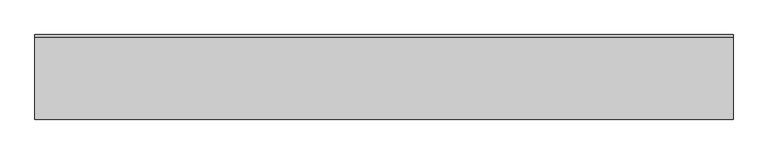
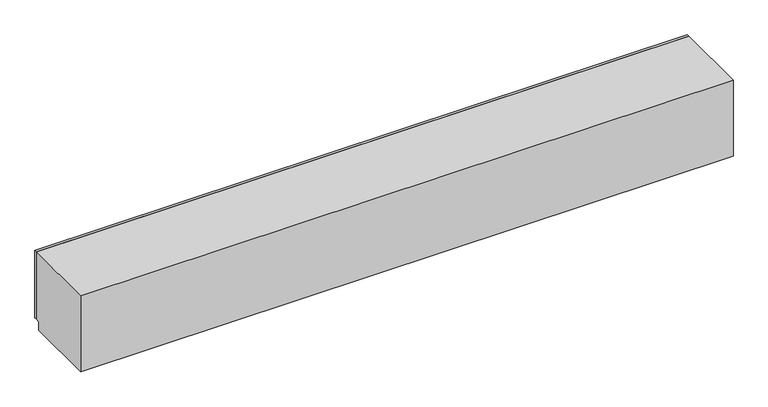
"""IFC4 building model written with IfcOpenShell, lengths in millimetres: furniture geometry, OD_CW_Base Cabinet : OD_CW_Base Cabinet."""

from ifc_helpers import new_model, si_unit, frame, origin, place, context, project, spatial, polyline, outline, extrude, source, transform, mapped, element, save


def furniture_3adb2dd1(model_context):
    return source(origin(), model_context, "Body", "SweptSolid", [
        extrude(outline(polyline([(18.7377049, 228.6), (18.7377049, 254.0), (7146.0765875, 254.0), (7146.0765875, 228.6), (18.7377049, 228.6)])), frame((0.0, 0.0, 101.6), z_axis=(0.0, 0.0, 1.0), x_axis=(1.0, 0.0, 0.0)), (0.0, 0.0, 1.0), 774.7),
        extrude(outline(polyline([(228.6, 876.3), (228.6, 101.6), (177.8, 101.6), (177.8, 0.0), (-609.6, 0.0), (-609.6, 876.3), (228.6, 876.3)])), frame((18.7377049, 0.0, 0.0), z_axis=(1.0, 0.0, 0.0), x_axis=(0.0, 1.0, 0.0)), (0.0, 0.0, 1.0), 7127.3388826),
    ])


if __name__ == "__main__":
    model = new_model("IFC4")
    model_context = context("Model", 3, world=origin())
    ifc_project = project(units=[si_unit("LENGTHUNIT", "METRE", prefix="MILLI")], contexts=[model_context])
    site = spatial("IfcSite", under=ifc_project)
    building = spatial("IfcBuilding", under=site)
    placement = place(None, origin())
    furniture_shape = furniture_3adb2dd1(model_context)
    element("IfcFurniture", 1, ObjectType="OD_CW_Base Cabinet : OD_CW_Base Cabinet", at=placement, inside=building, context=model_context, shape_type="MappedRepresentation", body=[
        mapped(furniture_shape, transform((0.0, 0.0, 0.0), x_axis=(1.0, 0.0, 0.0), y_axis=(0.0, 1.0, 0.0), z_axis=(0.0, 0.0, 1.0))),
    ])
    save(model, "model.ifc")

# Revit data of these elements
# Type "OD_CW_Base Cabinet : OD_CW_Base Cabinet"
#   OD_CW_Width [instance default] = 2' - 10"
#   OD_CW_Length [instance default] = 8' - 0"
#   OD_CW_Height [instance default] = 2' - 3"
#   Depth = 2' - 0"
#   Height = 3' - 0"
#   Width = 4' - 0"
#   OD_CW_Material_Front Panel [instance default] = none
#   OD_CW_Material_Body [instance default] = none
# Element 1 (IfcFurniture, "OD_CW_Base Cabinet : OD_CW_Base Cabinet")
#   OD_CW_Length = 23' - 4.60389"
#   OD_CW_Height = 2' - 10 1/2"
#   Materials on its faces: "CASEWORK"
# Materials
#   "CASEWORK": class "Generic", colour RGB 181 181 181, transparency 0, Cost = 0
